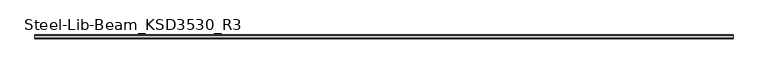
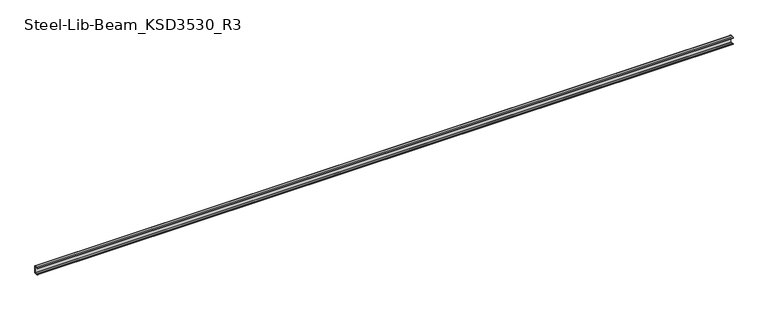
"""IFC4 building model written with IfcOpenShell, lengths in millimetres: beam geometry, Steel-Lib-Beam_KSD3530_R3 : BMS291_C-150×75x20x4.5."""

from ifc_helpers import new_model, si_unit, point, frame, frame_2d, origin, place, context, project, spatial, polyline, circle_curve, trimmed, segment, composite_curve, outline, extrude, source, transform, mapped, element, save


def steel_lib_beam_ksd3530_r3_b8669efc(model_context):
    return source(origin(), model_context, "Body", "SweptSolid", [
        extrude(outline(composite_curve([segment(trimmed(circle_curve(frame_2d((-41.0, 66.0)), 9.0), [point((-50.0, 66.0))], [point((-41.0, 75.0))], False, "CARTESIAN"), True, "CONTINUOUS"), segment(polyline([(-41.0, 75.0), (16.0, 75.0)]), True, "CONTINUOUS"), segment(trimmed(circle_curve(frame_2d((16.0, 66.0)), 9.0), [point((16.0, 75.0))], [point((25.0, 66.0))], False, "CARTESIAN"), True, "CONTINUOUS"), segment(polyline([(25.0, 66.0), (25.0, -66.0)]), True, "CONTINUOUS"), segment(trimmed(circle_curve(frame_2d((16.0, -66.0)), 9.0), [point((25.0, -66.0))], [point((16.0, -75.0))], False, "CARTESIAN"), True, "CONTINUOUS"), segment(polyline([(16.0, -75.0), (-41.0, -75.0)]), True, "CONTINUOUS"), segment(trimmed(circle_curve(frame_2d((-41.0, -66.0)), 9.0), [point((-41.0, -75.0))], [point((-50.0, -66.0))], False, "CARTESIAN"), True, "CONTINUOUS"), segment(polyline([(-50.0, -66.0), (-50.0, -55.0), (-45.5, -55.0), (-45.5, -66.0)]), True, "CONTINUOUS"), segment(trimmed(circle_curve(frame_2d((-41.0, -66.0)), 4.5), [point((-45.5, -66.0))], [point((-41.0, -70.5))], True, "CARTESIAN"), True, "CONTINUOUS"), segment(polyline([(-41.0, -70.5), (16.0, -70.5)]), True, "CONTINUOUS"), segment(trimmed(circle_curve(frame_2d((16.0, -66.0)), 4.5), [point((16.0, -70.5))], [point((20.5, -66.0))], True, "CARTESIAN"), True, "CONTINUOUS"), segment(polyline([(20.5, -66.0), (20.5, 66.0)]), True, "CONTINUOUS"), segment(trimmed(circle_curve(frame_2d((16.0, 66.0)), 4.5), [point((20.5, 66.0))], [point((16.0, 70.5))], True, "CARTESIAN"), True, "CONTINUOUS"), segment(polyline([(16.0, 70.5), (-41.0, 70.5)]), True, "CONTINUOUS"), segment(trimmed(circle_curve(frame_2d((-41.0, 66.0)), 4.5), [point((-41.0, 70.5))], [point((-45.5, 66.0))], True, "CARTESIAN"), True, "CONTINUOUS"), segment(polyline([(-45.5, 66.0), (-45.5, 55.0), (-50.0, 55.0), (-50.0, 66.0)]), True, "CONTINUOUS")], self_intersect=False)), frame((-6620.5, 0.0, 0.0), z_axis=(1.0, 0.0, 0.0), x_axis=(0.0, 1.0, 0.0)), (0.0, 0.0, 1.0), 13241.0),
    ])


if __name__ == "__main__":
    model = new_model("IFC4")
    model_context = context("Model", 3, world=origin())
    ifc_project = project(units=[si_unit("LENGTHUNIT", "METRE", prefix="MILLI")], contexts=[model_context])
    site = spatial("IfcSite", under=ifc_project)
    building = spatial("IfcBuilding", under=site)
    placement = place(None, origin())
    steel_lib_beam_ksd3530_r3_shape = steel_lib_beam_ksd3530_r3_b8669efc(model_context)
    element("IfcBeam", 1, ObjectType="Steel-Lib-Beam_KSD3530_R3 : BMS291_C-150×75x20x4.5", at=placement, inside=building, context=model_context, shape_type="MappedRepresentation", body=[
        mapped(steel_lib_beam_ksd3530_r3_shape, transform((0.0, 0.0, 0.0), x_axis=(1.0, 0.0, 0.0), y_axis=(0.0, 1.0, 0.0), z_axis=(0.0, 0.0, 1.0))),
    ])
    save(model, "model.ifc")

# Revit data of these elements
# Type "Steel-Lib-Beam_KSD3530_R3 : BMS291_C-150×75x20x4.5"
#   Keynote = "C-150×75x20x4.5"
#   SteelWeight = "Light"
#   x = 0.0250 m
#   t1 = 0.0090 m
#   t = 0.0045 m
#   Surface Area = 0.629834 m²/m
#   Section Area = 13.9688 cm²
#   Mass per Unit Length = 10.9655 kg/m
#   C = 0.0200 m
#   A = 0.0750 m
#   Length [instance default] = 1.5000 m
#   H = 0.1500 m
#   hec_material4 [instance default] = none
#   hec_material3 [instance default] = none
#   hec_material2 [instance default] = none
#   hec_material1 [instance default] = none
#   Structural Material [instance default] = Metal - Steel - Light Gauge
#   Assembly Code = ""
# Element 1 (IfcBeam, "Steel-Lib-Beam_KSD3530_R3 : BMS291_C-150×75x20x4.5")
#   Structural Material = none
# Materials
#   "Metal - Steel - Light Gauge": class "Metal", colour RGB 247 247 247, transparency 0
